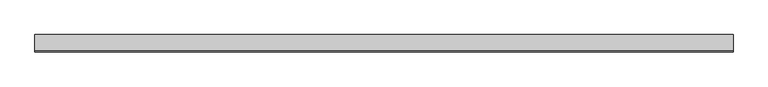
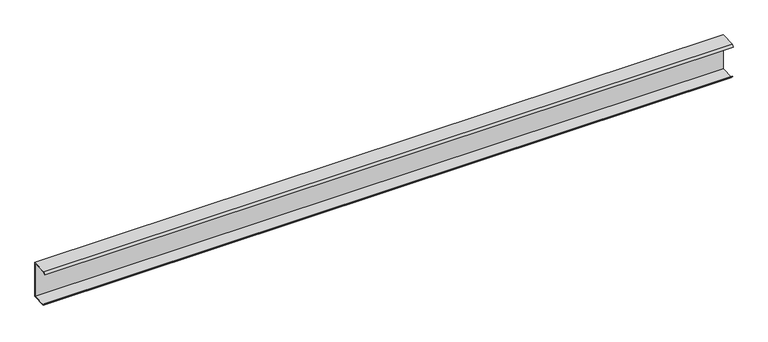
"""IFC4 building model written with IfcOpenShell, lengths in millimetres: proxy geometry, Generic Models 7:Generic Models 1:8:Generic Models 1:8 : Generic Models 7:Generic Models 1:337419:16 : Generic Models 7:Generic Models 1:8:Generic Models 1:8 : Generic Models 7:Generic Models 1:337419:315935."""

from ifc_helpers import new_model, si_unit, frame, origin, place, context, project, spatial, polyline, outline, extrude, source, transform, mapped, element, save


def generic_models_91a6796d(model_context):
    return source(origin(), model_context, "Body", "SweptSolid", [
        extrude(outline(polyline([(-536666.5741925, 10091.6100484), (-536557.2913841, 10096.1634988), (-536557.2913841, 9841.9431083), (-536658.1992191, 9837.7386152), (-536671.0412281, 9851.8093403), (-536668.9720791, 9853.6978023), (-536656.9902199, 9840.5695257), (-536560.0695091, 9844.6078886), (-536560.0695091, 10093.267208), (-536665.1338836, 10088.8895258), (-536675.9820842, 10074.8099966), (-536678.2011602, 10076.5197826), (-536666.5741925, 10091.6100484)])), frame((591306.0367242, 0.0, 0.0), z_axis=(1.0, 0.0, 0.0), x_axis=(0.0, 1.0, 0.0)), (0.0, 0.0, 1.0), 4876.8),
    ])


if __name__ == "__main__":
    model = new_model("IFC4")
    model_context = context("Model", 3, world=origin())
    ifc_project = project(units=[si_unit("LENGTHUNIT", "METRE", prefix="MILLI")], contexts=[model_context])
    site = spatial("IfcSite", under=ifc_project)
    building = spatial("IfcBuilding", under=site)
    placement = place(None, origin())
    generic_models_shape = generic_models_91a6796d(model_context)
    element("IfcBuildingElementProxy", 1, Name="Generic Models 7:Generic Models 1:8:Generic Models 1:8 : Generic Models 7:Generic Models 1:337419:16 : Generic Models 7:Generic Models 1:8:Generic Models 1:8 : Generic Models 7:Generic Models 1:337419:315935", ObjectType="Generic Models 7:Generic Models 1:8:Generic Models 1:8 : Generic Models 7:Generic Models 1:337419:16 : Generic Models 7:Generic Models 1:8:Generic Models 1:8 : Generic Models 7:Generic Models 1:337419:315935", at=placement, inside=building, context=model_context, shape_type="MappedRepresentation", body=[
        mapped(generic_models_shape, transform((0.0, 0.0, 0.0), x_axis=(1.0, 0.0, 0.0), y_axis=(0.0, 1.0, 0.0), z_axis=(0.0, 0.0, 1.0))),
    ])
    save(model, "model.ifc")

# Revit data of these elements
# Type "Generic Models 7:Generic Models 1:8:Generic Models 1:8 : Generic Models 7:Generic Models 1:337419:16 : Generic Models 7:Generic Models 1:8:Generic Models 1:8 : Generic Models 7:Generic Models 1:337419:315935"
#   NameOverride = "Generic Models 7:Generic Models 1:8:Generic Models 1:8 : Generic Models 7:Generic Models 1:337419:315935"
#   ObjectTypeOverride = "Generic Models 1:8 : Generic Models 7:Generic Models 1:337419"
#   Reference = "Generic Models 1"
#   Tag = "315935"
# Element 1 (IfcBuildingElementProxy, "Generic Models 7:Generic Models 1:8:Generic Models 1:8 : Generic Models 7:Generic Models 1:337419:16 : Generic Models 7:Generic Models 1:8:Generic Models 1:8 : Generic Models 7:Generic Models 1:337419:315935")
#   Materials on its faces: "EAVE STRUCT - SEE STRUCT. DWGS."
# Materials
#   "EAVE STRUCT - SEE STRUCT. DWGS.": class "Unassigned", colour RGB 210 209 208, transparency 0, Cost = 0
